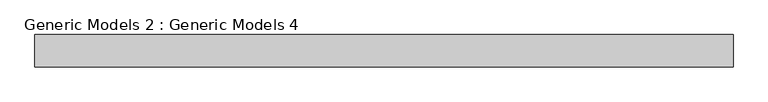
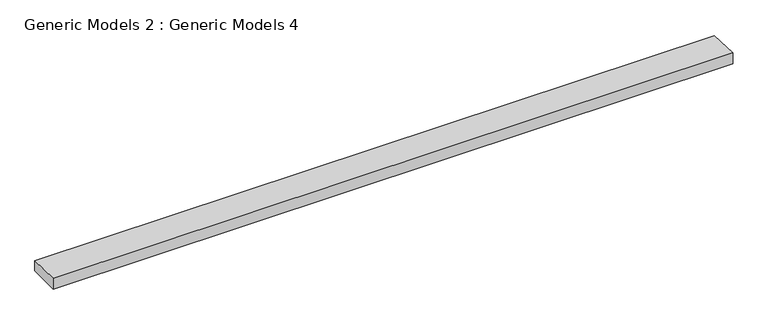
"""IFC4 building model written with IfcOpenShell, lengths in millimetres: proxy geometry, Generic Models 2 : Generic Models 4."""

from ifc_helpers import new_model, si_unit, frame, origin, place, context, project, spatial, polyline, outline, extrude, source, transform, mapped, element, save


def generic_models_2_generic_models_4_8d8120a8(model_context):
    return source(origin(), model_context, "Body", "SweptSolid", [
        extrude(outline(polyline([(-24416.1512987, 126208.263557), (-24703.0614163, 126208.263557), (-24703.0614163, 126312.7712179), (-24416.1512987, 126306.7939238), (-24416.1512987, 126208.263557)])), frame((2196.9263704, 0.0, 0.0), z_axis=(1.0, 0.0, 0.0), x_axis=(0.0, 1.0, 0.0)), (0.0, 0.0, 1.0), 6189.931498),
    ])


if __name__ == "__main__":
    model = new_model("IFC4")
    model_context = context("Model", 3, world=origin())
    ifc_project = project(units=[si_unit("LENGTHUNIT", "METRE", prefix="MILLI")], contexts=[model_context])
    site = spatial("IfcSite", under=ifc_project)
    building = spatial("IfcBuilding", under=site)
    placement = place(None, origin())
    generic_models_2_generic_models_4_shape = generic_models_2_generic_models_4_8d8120a8(model_context)
    element("IfcBuildingElementProxy", 1, Name="Generic Models 2 : Generic Models 4", ObjectType="Generic Models 2 : Generic Models 4", at=placement, inside=building, context=model_context, shape_type="MappedRepresentation", body=[
        mapped(generic_models_2_generic_models_4_shape, transform((0.0, 0.0, 0.0), x_axis=(1.0, 0.0, 0.0), y_axis=(0.0, 1.0, 0.0), z_axis=(0.0, 0.0, 1.0))),
    ])
    save(model, "model.ifc")

# Revit data of these elements
# Element 1 (IfcBuildingElementProxy, "Generic Models 2 : Generic Models 4")
#   Materials on its faces: "_TAPERED 2X BLOCKING (1% SLOPE) - SLOPED TOWARD DRAINS (SEE ROOF PLAN)"
# Materials
#   "_TAPERED 2X BLOCKING (1% SLOPE) - SLOPED TOWARD DRAINS (SEE ROOF PLAN)": class "Generic", colour RGB 177 130 114, transparency 0, Cost = 0
